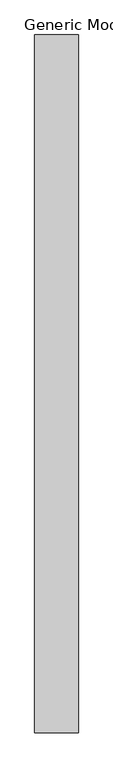
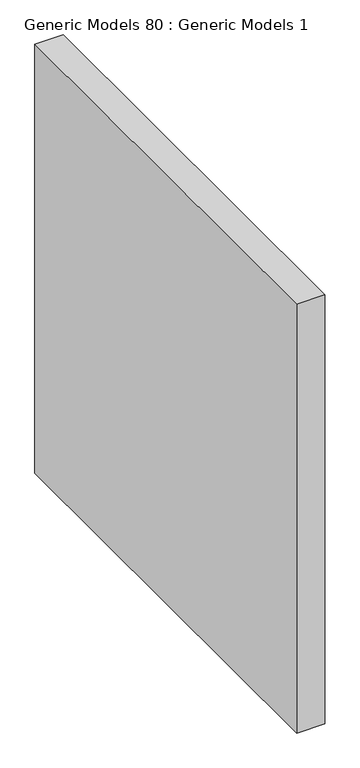
"""IFC4 building model written with IfcOpenShell, lengths in millimetres: proxy geometry, Generic Models 80 : Generic Models 1."""

from ifc_helpers import new_model, si_unit, frame, origin, place, context, project, spatial, polyline, outline, extrude, source, transform, mapped, element, save


def generic_models_80_generic_models_1_8b1a960f(model_context):
    return source(origin(), model_context, "Body", "SweptSolid", [
        extrude(outline(polyline([(48556.8625, 0.0), (48480.6625, 0.0), (48480.6625, 1219.2), (48556.8625, 1219.2), (48556.8625, 0.0)])), frame((0.0, 0.0, 1264.512912), z_axis=(0.0, 0.0, 1.0), x_axis=(1.0, 0.0, 0.0)), (0.0, 0.0, 1.0), 1219.2),
    ])


if __name__ == "__main__":
    model = new_model("IFC4")
    model_context = context("Model", 3, world=origin())
    ifc_project = project(units=[si_unit("LENGTHUNIT", "METRE", prefix="MILLI")], contexts=[model_context])
    site = spatial("IfcSite", under=ifc_project)
    building = spatial("IfcBuilding", under=site)
    placement = place(None, origin())
    generic_models_80_generic_models_1_shape = generic_models_80_generic_models_1_8b1a960f(model_context)
    element("IfcBuildingElementProxy", 1, Name="Generic Models 80 : Generic Models 1", ObjectType="Generic Models 80 : Generic Models 1", at=placement, inside=building, context=model_context, shape_type="MappedRepresentation", body=[
        mapped(generic_models_80_generic_models_1_shape, transform((0.0, 0.0, 0.0), x_axis=(1.0, 0.0, 0.0), y_axis=(0.0, 1.0, 0.0), z_axis=(0.0, 0.0, 1.0))),
    ])
    save(model, "model.ifc")

# Revit data of these elements
# Element 1 (IfcBuildingElementProxy, "Generic Models 80 : Generic Models 1")
#   Materials on its faces: "SOUND BATT. INSULATION (THICKNESS TO MATCH WALL DEPTH)"
# Materials
#   "SOUND BATT. INSULATION (THICKNESS TO MATCH WALL DEPTH)": class "Unassigned", colour RGB 255 255 255, transparency 0, Cost = 0
